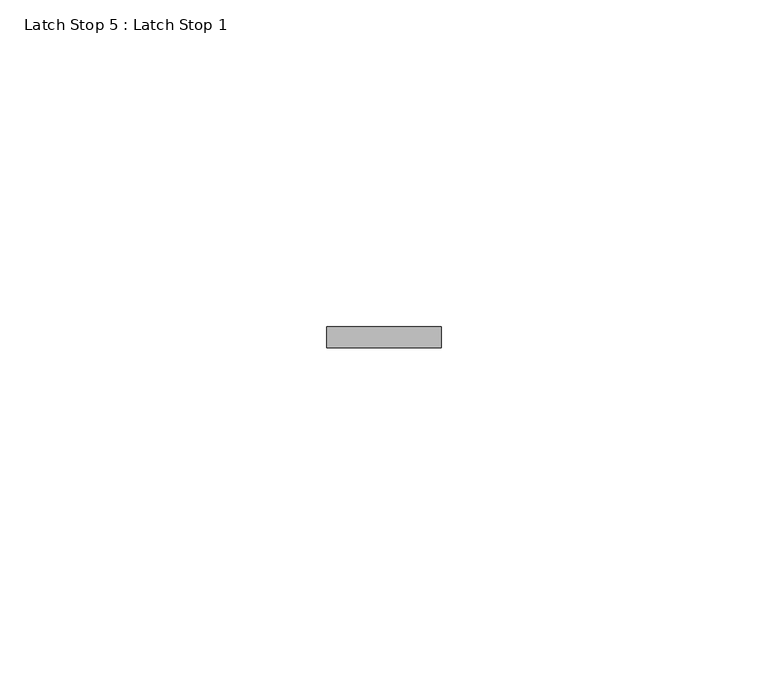
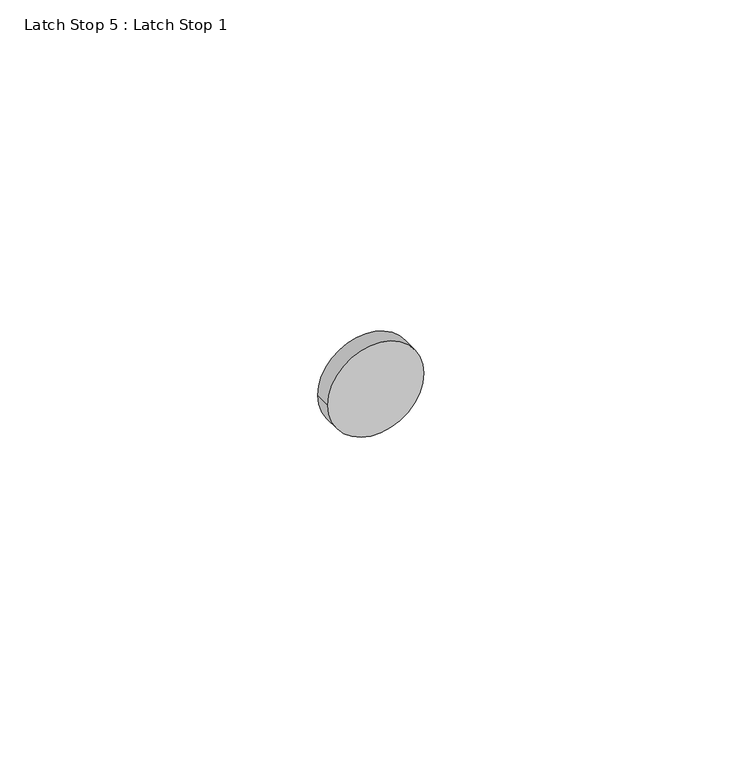
"""IFC4 building model written with IfcOpenShell, lengths in millimetres: proxy geometry, Latch Stop 5 : Latch Stop 1."""

from ifc_helpers import new_model, si_unit, point, frame, frame_2d, origin, place, context, project, spatial, circle_curve, trimmed, segment, composite_curve, outline, extrude, source, transform, mapped, element, save


def latch_stop_5_latch_stop_1_b083edd1(model_context):
    return source(origin(), model_context, "Body", "SweptSolid", [
        extrude(outline(composite_curve([segment(trimmed(circle_curve(frame_2d((1066.8, 587312.7185739)), 8.73125), [point((1066.8, 587303.9873239))], [point((1066.8, 587321.4498239))], False, "CARTESIAN"), True, "CONTINUOUS"), segment(trimmed(circle_curve(frame_2d((1066.8, 587312.7185739)), 8.73125), [point((1066.8, 587321.4498239))], [point((1066.8, 587303.9873239))], False, "CARTESIAN"), True, "CONTINUOUS")], self_intersect=False)), frame((0.0, -532842.5413841, 0.0), z_axis=(0.0, 1.0, 0.0), x_axis=(0.0, 0.0, 1.0)), (0.0, 0.0, 1.0), 3.175),
    ])


if __name__ == "__main__":
    model = new_model("IFC4")
    model_context = context("Model", 3, world=origin())
    ifc_project = project(units=[si_unit("LENGTHUNIT", "METRE", prefix="MILLI")], contexts=[model_context])
    site = spatial("IfcSite", under=ifc_project)
    building = spatial("IfcBuilding", under=site)
    placement = place(None, origin())
    latch_stop_5_latch_stop_1_shape = latch_stop_5_latch_stop_1_b083edd1(model_context)
    element("IfcBuildingElementProxy", 1, Name="Latch Stop 5 : Latch Stop 1", ObjectType="Latch Stop 5 : Latch Stop 1", at=placement, inside=building, context=model_context, shape_type="MappedRepresentation", body=[
        mapped(latch_stop_5_latch_stop_1_shape, transform((0.0, 0.0, 0.0), x_axis=(1.0, 0.0, 0.0), y_axis=(0.0, 1.0, 0.0), z_axis=(0.0, 0.0, 1.0))),
    ])
    save(model, "model.ifc")

# Revit data of these elements
# Element 1 (IfcBuildingElementProxy, "Latch Stop 5 : Latch Stop 1")
#   Materials on its faces: "GALV. GATE LATCH"
# Materials
#   "GALV. GATE LATCH": class "Metal", colour RGB 189 187 185, transparency 0, Description = "Carbon steel", Cost = 0
